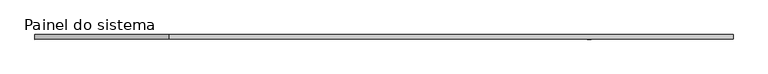
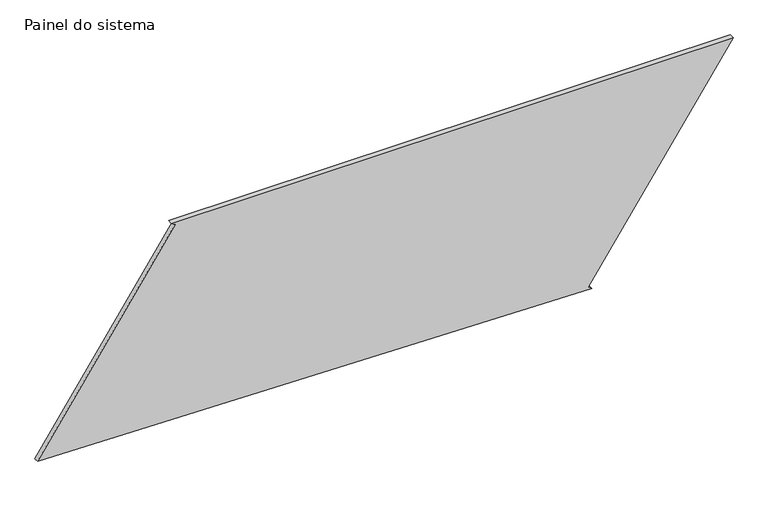
"""IFC4 building model written with IfcOpenShell, lengths in millimetres: plate geometry, Painel do sistema : Envidraçado."""

import ifcopenshell
import ifcopenshell.guid

model = None  # the IFC model being written
_history = None  # IfcOwnerHistory: only IFC2X3 demands one
_inside = {}  # id of a spatial element -> (the spatial element, [elements in it])
_under = {}  # id of a project, library or spatial element -> (it, [spatial elements below it])
_declared = {}  # id of a project -> (the project, [libraries it declares])
_typed = {}  # id of a type object -> (the type object, [elements of that type])
_made_of = {}  # id of a material, layer set ... -> (it, [elements and type objects made of it])


def new_model(schema):
    """Start an empty IFC model of exactly this schema.

    Asked for "IFC4X3", IfcOpenShell would pick the latest addendum, in which some entities
    have other attributes; the version numbers below select the first issue.
    IFC2X3 requires an IfcOwnerHistory on every rooted entity: one is made here for all.
    """
    global model, _history
    if schema == "IFC4X3":
        model = ifcopenshell.file(schema_version=(4, 3, 0, 0))
    else:
        model = ifcopenshell.file(schema=schema)
    _inside.clear()
    _under.clear()
    _declared.clear()
    _typed.clear()
    _made_of.clear()
    _history = None
    if model.schema == "IFC2X3":
        org = make("IfcOrganization", Name="unknown")
        user = make(
            "IfcPersonAndOrganization",
            ThePerson=make("IfcPerson", FamilyName="unknown"),
            TheOrganization=org,
        )
        app = make(
            "IfcApplication",
            ApplicationDeveloper=org,
            Version="unknown",
            ApplicationFullName="unknown",
            ApplicationIdentifier="unknown",
        )
        _history = make(
            "IfcOwnerHistory",
            OwningUser=user,
            OwningApplication=app,
            ChangeAction="ADDED",
            CreationDate=0,
        )
    return model


def make(cls, **values):
    """One entity of the class cls with the attributes given. An attribute that is None is left unset."""
    return model.create_entity(
        cls, **{name: value for name, value in values.items() if value is not None}
    )


def rooted(cls, **values):
    """An entity with a GlobalId (a new one), such as an element, a storey or a relation."""
    return make(cls, GlobalId=ifcopenshell.guid.new(), OwnerHistory=_history, **values)


def si_unit(unit_type, name, prefix=None):
    """IfcSIUnit, for example si_unit("LENGTHUNIT", "METRE", prefix="MILLI")."""
    return make("IfcSIUnit", UnitType=unit_type, Prefix=prefix, Name=name)


def assignment(units):
    """IfcUnitAssignment: the units of a project."""
    return None if units is None else make("IfcUnitAssignment", Units=units)


def point(xyz):
    """IfcCartesianPoint."""
    return None if xyz is None else make("IfcCartesianPoint", Coordinates=xyz)


def direction(xyz):
    """IfcDirection."""
    return None if xyz is None else make("IfcDirection", DirectionRatios=xyz)


def frame(location, z_axis=None, x_axis=None):
    """IfcAxis2Placement3D, a coordinate frame: its origin and axes. An axis left out is left unset."""
    return make(
        "IfcAxis2Placement3D",
        Location=point(location),
        Axis=direction(z_axis),
        RefDirection=direction(x_axis),
    )


def origin():
    """The frame at (0, 0, 0) with its axes left unset."""
    return frame((0.0, 0.0, 0.0))


def place(relative_to, where):
    """IfcLocalPlacement: puts the frame where relative to a parent placement (None: the world)."""
    return make(
        "IfcLocalPlacement", PlacementRelTo=relative_to, RelativePlacement=where
    )


def context(
    kind, dimensions, precision=None, world=None, true_north=None, identifier=None
):
    """IfcGeometricRepresentationContext, for example the 3D "Model" context."""
    return make(
        "IfcGeometricRepresentationContext",
        ContextIdentifier=identifier,
        ContextType=kind,
        CoordinateSpaceDimension=dimensions,
        Precision=precision,
        WorldCoordinateSystem=world,
        TrueNorth=true_north,
    )


def project(units=None, contexts=None):
    """IfcProject with its units and contexts."""
    return rooted(
        "IfcProject",
        Name="project",
        RepresentationContexts=contexts,
        UnitsInContext=assignment(units),
    )


def spatial(cls, under=None, at=None, **own):
    """A site, building, storey or space (cls), placed at a placement, below another one or the project."""
    s = rooted(cls, ObjectPlacement=at, **own)
    if under is not None:
        _under.setdefault(under.id(), (under, []))[1].append(s)
    return s


def polyline(points):
    """IfcPolyline through the points."""
    return make("IfcPolyline", Points=[point(p) for p in points])


def outline(outer, holes=None, kind="AREA"):
    """IfcArbitraryClosedProfileDef: a profile drawn as a closed curve; with holes, ...WithVoids."""
    if holes is None:
        return make("IfcArbitraryClosedProfileDef", ProfileType=kind, OuterCurve=outer)
    return make(
        "IfcArbitraryProfileDefWithVoids",
        ProfileType=kind,
        OuterCurve=outer,
        InnerCurves=holes,
    )


def extrude(swept, where, along, depth):
    """IfcExtrudedAreaSolid: the profile swept, set in the frame where, extruded along a direction by depth."""
    return make(
        "IfcExtrudedAreaSolid",
        SweptArea=swept,
        Position=where,
        ExtrudedDirection=direction(along),
        Depth=depth,
    )


def shape(context_of_items, identifier, shape_type, items):
    """IfcShapeRepresentation: the items that make up one representation, for example the "Body"."""
    return make(
        "IfcShapeRepresentation",
        ContextOfItems=context_of_items,
        RepresentationIdentifier=identifier,
        RepresentationType=shape_type,
        Items=items,
    )


def source(mapping_origin, context_of_items, identifier, shape_type, items):
    """IfcRepresentationMap: a shape defined once, which mapped items show again and again."""
    return make(
        "IfcRepresentationMap",
        MappingOrigin=mapping_origin,
        MappedRepresentation=shape(context_of_items, identifier, shape_type, items),
    )


def transform(
    local_origin,
    x_axis=None,
    y_axis=None,
    z_axis=None,
    scale=None,
    scale2=None,
    scale3=None,
    uniform=True,
):
    """IfcCartesianTransformationOperator3D, or its non-uniform kind. x_axis, y_axis, z_axis: its Axis1, 2, 3."""
    if uniform:
        return make(
            "IfcCartesianTransformationOperator3D",
            Axis1=direction(x_axis),
            Axis2=direction(y_axis),
            LocalOrigin=point(local_origin),
            Scale=scale,
            Axis3=direction(z_axis),
        )
    return make(
        "IfcCartesianTransformationOperator3DnonUniform",
        Axis1=direction(x_axis),
        Axis2=direction(y_axis),
        LocalOrigin=point(local_origin),
        Scale=scale,
        Axis3=direction(z_axis),
        Scale2=scale2,
        Scale3=scale3,
    )


def mapped(mapping_source, mapping_target):
    """IfcMappedItem: shows the shape of a source again, moved by a transform."""
    return make(
        "IfcMappedItem", MappingSource=mapping_source, MappingTarget=mapping_target
    )


def made_of(thing, what):
    """Note that an element or type object is made of a material, layer set ...; save() writes the relation."""
    if what is not None:
        _made_of.setdefault(what.id(), (what, []))[1].append(thing)
    return thing


def element(
    cls,
    number,
    at=None,
    inside=None,
    cuts=None,
    type_object=None,
    material=None,
    context=None,
    identifier="Body",
    shape_type=None,
    held_by="IfcProductDefinitionShape",
    body=None,
    shapes=None,
    **own,
):
    """One element of the class cls, such as IfcWall. Its Tag is "e" and its number.

    at: its placement. inside: the storey or other place that contains it. cuts: it is an
    opening in that element (IfcRelVoidsElement). A single representation is given by context,
    identifier, shape_type and body (its items); several are given by shapes. held_by: the class
    of the entity that holds the representations. save() writes the other relations.
    """
    e = rooted(cls, Tag="e%d" % number, ObjectPlacement=at, **own)
    if body is not None:
        shapes = [shape(context, identifier, shape_type, body)]
    if shapes is not None:
        e.Representation = make(held_by, Representations=shapes)
    if inside is not None:
        _inside.setdefault(inside.id(), (inside, []))[1].append(e)
    if cuts is not None:
        rooted(
            "IfcRelVoidsElement", RelatingBuildingElement=cuts, RelatedOpeningElement=e
        )
    if type_object is not None:
        _typed.setdefault(type_object.id(), (type_object, []))[1].append(e)
    return made_of(e, material)


def aggregate(whole, parts):
    """IfcRelAggregates: a whole, such as a stair, and the parts it consists of."""
    return rooted("IfcRelAggregates", RelatingObject=whole, RelatedObjects=parts)


def save(model, path):
    """Write the relations noted so far, then the file.

    IfcRelAggregates (storeys below a building ...), IfcRelContainedInSpatialStructure (elements
    in a storey), IfcRelDefinesByType, IfcRelAssociatesMaterial and IfcRelDeclares: one each for
    every whole, place, type object, material and project.
    """
    for whole, parts in _under.values():
        aggregate(whole, parts)
    for where, things in _inside.values():
        rooted(
            "IfcRelContainedInSpatialStructure",
            RelatedElements=things,
            RelatingStructure=where,
        )
    for kind, things in _typed.values():
        rooted("IfcRelDefinesByType", RelatedObjects=things, RelatingType=kind)
    for what, things in _made_of.values():
        rooted("IfcRelAssociatesMaterial", RelatedObjects=things, RelatingMaterial=what)
    for by, libraries in _declared.values():
        rooted("IfcRelDeclares", RelatingContext=by, RelatedDefinitions=libraries)
    model.write(path)


def painel_do_sistema_7887c898(model_context):
    return source(origin(), model_context, "Body", "SweptSolid", [
        extrude(outline(polyline([(0.0, 1132.1256958), (14.052453, 1111.4489319), (1184.3317252, 1906.800396), (1184.3317252, -1173.5038412), (1170.2792722, -1152.8270773), (60.8837577, -1906.800396), (0.0, 1132.1256958)])), frame((0.0, 24.5, 0.0), z_axis=(0.0, 1.0, 0.0), x_axis=(0.0, 0.0, 1.0)), (0.0, 0.0, 1.0), 25.0),
    ])


if __name__ == "__main__":
    model = new_model("IFC4")
    model_context = context("Model", 3, world=origin())
    ifc_project = project(units=[si_unit("LENGTHUNIT", "METRE", prefix="MILLI")], contexts=[model_context])
    site = spatial("IfcSite", under=ifc_project)
    building = spatial("IfcBuilding", under=site)
    placement = place(None, origin())
    painel_do_sistema_shape = painel_do_sistema_7887c898(model_context)
    element("IfcPlate", 1, ObjectType="Painel do sistema : Envidraçado", at=placement, inside=building, context=model_context, shape_type="MappedRepresentation", body=[
        mapped(painel_do_sistema_shape, transform((0.0, 0.0, 0.0), x_axis=(1.0, 0.0, 0.0), y_axis=(0.0, 1.0, 0.0), z_axis=(0.0, 0.0, 1.0))),
    ])
    save(model, "model.ifc")

# Revit data of these elements
# Type "Painel do sistema : Envidraçado"
#   Construction Type Id = "GSP4R"
#   Analytic Construction = "Vidraça única Pilkington 1/8 pol"
#   Visual Light Transmittance = 0.9
#   Solar Heat Gain Coefficient = 0.86
#   Heat Transfer Coefficient (U) = 6.7069 W/(m²·K)
# Element 1 (IfcPlate, "Painel do sistema : Envidraçado")
#   Materials on its faces: "Vidro"
# Materials
#   "Vidro": class "Vidro", colour RGB 0 128 192, transparency 0.9, Description = "Vidro de sílica", Cost = 0
